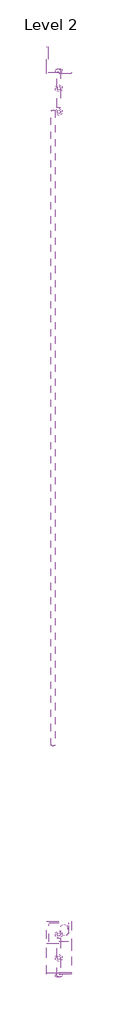
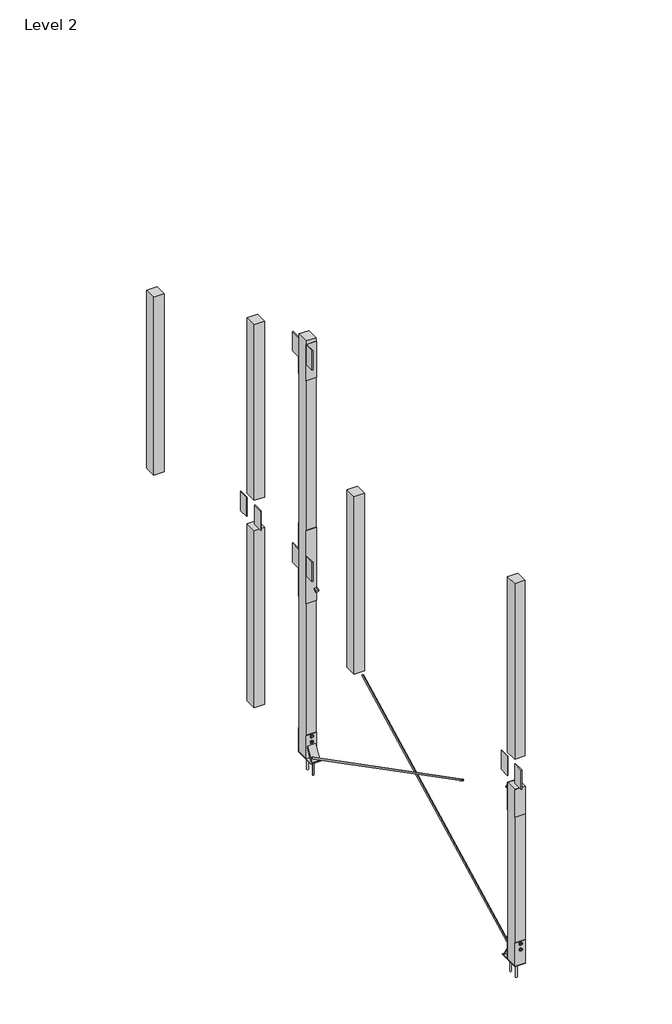
# One storey: 22 proxies, 1 column.
"""IFC4 building model written with IfcOpenShell, lengths in millimetres."""

import ifcopenshell
import ifcopenshell.guid

model = None  # the IFC model being written
_history = None  # IfcOwnerHistory: only IFC2X3 demands one
_inside = {}  # id of a spatial element -> (the spatial element, [elements in it])
_under = {}  # id of a project, library or spatial element -> (it, [spatial elements below it])
_declared = {}  # id of a project -> (the project, [libraries it declares])
_typed = {}  # id of a type object -> (the type object, [elements of that type])
_made_of = {}  # id of a material, layer set ... -> (it, [elements and type objects made of it])


def new_model(schema):
    """Start an empty IFC model of exactly this schema.

    Asked for "IFC4X3", IfcOpenShell would pick the latest addendum, in which some entities
    have other attributes; the version numbers below select the first issue.
    IFC2X3 requires an IfcOwnerHistory on every rooted entity: one is made here for all.
    """
    global model, _history
    if schema == "IFC4X3":
        model = ifcopenshell.file(schema_version=(4, 3, 0, 0))
    else:
        model = ifcopenshell.file(schema=schema)
    _inside.clear()
    _under.clear()
    _declared.clear()
    _typed.clear()
    _made_of.clear()
    _history = None
    if model.schema == "IFC2X3":
        org = make("IfcOrganization", Name="unknown")
        user = make(
            "IfcPersonAndOrganization",
            ThePerson=make("IfcPerson", FamilyName="unknown"),
            TheOrganization=org,
        )
        app = make(
            "IfcApplication",
            ApplicationDeveloper=org,
            Version="unknown",
            ApplicationFullName="unknown",
            ApplicationIdentifier="unknown",
        )
        _history = make(
            "IfcOwnerHistory",
            OwningUser=user,
            OwningApplication=app,
            ChangeAction="ADDED",
            CreationDate=0,
        )
    return model


def make(cls, **values):
    """One entity of the class cls with the attributes given. An attribute that is None is left unset."""
    return model.create_entity(
        cls, **{name: value for name, value in values.items() if value is not None}
    )


def rooted(cls, **values):
    """An entity with a GlobalId (a new one), such as an element, a storey or a relation."""
    return make(cls, GlobalId=ifcopenshell.guid.new(), OwnerHistory=_history, **values)


def si_unit(unit_type, name, prefix=None):
    """IfcSIUnit, for example si_unit("LENGTHUNIT", "METRE", prefix="MILLI")."""
    return make("IfcSIUnit", UnitType=unit_type, Prefix=prefix, Name=name)


def assignment(units):
    """IfcUnitAssignment: the units of a project."""
    return None if units is None else make("IfcUnitAssignment", Units=units)


def point(xyz):
    """IfcCartesianPoint."""
    return None if xyz is None else make("IfcCartesianPoint", Coordinates=xyz)


def direction(xyz):
    """IfcDirection."""
    return None if xyz is None else make("IfcDirection", DirectionRatios=xyz)


def frame(location, z_axis=None, x_axis=None):
    """IfcAxis2Placement3D, a coordinate frame: its origin and axes. An axis left out is left unset."""
    return make(
        "IfcAxis2Placement3D",
        Location=point(location),
        Axis=direction(z_axis),
        RefDirection=direction(x_axis),
    )


def frame_2d(location, x_axis=None):
    """IfcAxis2Placement2D, a coordinate frame in the plane: its origin and x axis."""
    return make(
        "IfcAxis2Placement2D", Location=point(location), RefDirection=direction(x_axis)
    )


def origin():
    """The frame at (0, 0, 0) with its axes left unset."""
    return frame((0.0, 0.0, 0.0))


def place(relative_to, where):
    """IfcLocalPlacement: puts the frame where relative to a parent placement (None: the world)."""
    return make(
        "IfcLocalPlacement", PlacementRelTo=relative_to, RelativePlacement=where
    )


def context(
    kind, dimensions, precision=None, world=None, true_north=None, identifier=None
):
    """IfcGeometricRepresentationContext, for example the 3D "Model" context."""
    return make(
        "IfcGeometricRepresentationContext",
        ContextIdentifier=identifier,
        ContextType=kind,
        CoordinateSpaceDimension=dimensions,
        Precision=precision,
        WorldCoordinateSystem=world,
        TrueNorth=true_north,
    )


def project(units=None, contexts=None):
    """IfcProject with its units and contexts."""
    return rooted(
        "IfcProject",
        Name="project",
        RepresentationContexts=contexts,
        UnitsInContext=assignment(units),
    )


def spatial(cls, under=None, at=None, **own):
    """A site, building, storey or space (cls), placed at a placement, below another one or the project."""
    s = rooted(cls, ObjectPlacement=at, **own)
    if under is not None:
        _under.setdefault(under.id(), (under, []))[1].append(s)
    return s


def polyline(points):
    """IfcPolyline through the points."""
    return make("IfcPolyline", Points=[point(p) for p in points])


def circle_curve(where, radius):
    """IfcCircle in the frame where."""
    return make("IfcCircle", Position=where, Radius=radius)


def trimmed(basis, trim1, trim2, sense, master):
    """IfcTrimmedCurve: the piece of a basis curve between two trims."""
    return make(
        "IfcTrimmedCurve",
        BasisCurve=basis,
        Trim1=trim1,
        Trim2=trim2,
        SenseAgreement=sense,
        MasterRepresentation=master,
    )


def segment(curve, same_sense, transition):
    """IfcCompositeCurveSegment."""
    return make(
        "IfcCompositeCurveSegment",
        Transition=transition,
        SameSense=same_sense,
        ParentCurve=curve,
    )


def composite_curve(segments, self_intersect=None):
    """IfcCompositeCurve: segments joined end to end."""
    return make("IfcCompositeCurve", Segments=segments, SelfIntersect=self_intersect)


def outline(outer, holes=None, kind="AREA"):
    """IfcArbitraryClosedProfileDef: a profile drawn as a closed curve; with holes, ...WithVoids."""
    if holes is None:
        return make("IfcArbitraryClosedProfileDef", ProfileType=kind, OuterCurve=outer)
    return make(
        "IfcArbitraryProfileDefWithVoids",
        ProfileType=kind,
        OuterCurve=outer,
        InnerCurves=holes,
    )


def extrude(swept, where, along, depth):
    """IfcExtrudedAreaSolid: the profile swept, set in the frame where, extruded along a direction by depth."""
    return make(
        "IfcExtrudedAreaSolid",
        SweptArea=swept,
        Position=where,
        ExtrudedDirection=direction(along),
        Depth=depth,
    )


def faces_of(points, faces, orient=None, outer=None):
    """IfcFace entities. A face is a list of loops; a loop is a list of indices into points, from 0.

    orient and outer hold one flag for each loop. By default every Orientation is true, the
    first loop of a face is its IfcFaceOuterBound and the others are IfcFaceBound.
    """
    made = []
    for i, loops in enumerate(faces):
        bounds = []
        for j, loop in enumerate(loops):
            is_outer = j == 0 if outer is None else outer[i][j]
            bounds.append(
                make(
                    "IfcFaceOuterBound" if is_outer else "IfcFaceBound",
                    Bound=make("IfcPolyLoop", Polygon=[points[k] for k in loop]),
                    Orientation=True if orient is None else orient[i][j],
                )
            )
        made.append(make("IfcFace", Bounds=bounds))
    return made


def faceted_brep(points, faces, orient=None, outer=None, voids=None):
    """IfcFacetedBrep: a solid bounded by flat faces; with voids (closed shells), ...WithVoids."""
    shared = [point(p) for p in points]
    hull = make("IfcClosedShell", CfsFaces=faces_of(shared, faces, orient, outer))
    if voids is None:
        return make("IfcFacetedBrep", Outer=hull)
    return make(
        "IfcFacetedBrepWithVoids",
        Outer=hull,
        Voids=[
            make(cls, CfsFaces=faces_of(shared, fs, o, b)) for cls, fs, o, b in voids
        ],
    )


def shape(context_of_items, identifier, shape_type, items):
    """IfcShapeRepresentation: the items that make up one representation, for example the "Body"."""
    return make(
        "IfcShapeRepresentation",
        ContextOfItems=context_of_items,
        RepresentationIdentifier=identifier,
        RepresentationType=shape_type,
        Items=items,
    )


def source(mapping_origin, context_of_items, identifier, shape_type, items):
    """IfcRepresentationMap: a shape defined once, which mapped items show again and again."""
    return make(
        "IfcRepresentationMap",
        MappingOrigin=mapping_origin,
        MappedRepresentation=shape(context_of_items, identifier, shape_type, items),
    )


def transform(
    local_origin,
    x_axis=None,
    y_axis=None,
    z_axis=None,
    scale=None,
    scale2=None,
    scale3=None,
    uniform=True,
):
    """IfcCartesianTransformationOperator3D, or its non-uniform kind. x_axis, y_axis, z_axis: its Axis1, 2, 3."""
    if uniform:
        return make(
            "IfcCartesianTransformationOperator3D",
            Axis1=direction(x_axis),
            Axis2=direction(y_axis),
            LocalOrigin=point(local_origin),
            Scale=scale,
            Axis3=direction(z_axis),
        )
    return make(
        "IfcCartesianTransformationOperator3DnonUniform",
        Axis1=direction(x_axis),
        Axis2=direction(y_axis),
        LocalOrigin=point(local_origin),
        Scale=scale,
        Axis3=direction(z_axis),
        Scale2=scale2,
        Scale3=scale3,
    )


def mapped(mapping_source, mapping_target):
    """IfcMappedItem: shows the shape of a source again, moved by a transform."""
    return make(
        "IfcMappedItem", MappingSource=mapping_source, MappingTarget=mapping_target
    )


def made_of(thing, what):
    """Note that an element or type object is made of a material, layer set ...; save() writes the relation."""
    if what is not None:
        _made_of.setdefault(what.id(), (what, []))[1].append(thing)
    return thing


def element(
    cls,
    number,
    at=None,
    inside=None,
    cuts=None,
    type_object=None,
    material=None,
    context=None,
    identifier="Body",
    shape_type=None,
    held_by="IfcProductDefinitionShape",
    body=None,
    shapes=None,
    **own,
):
    """One element of the class cls, such as IfcWall. Its Tag is "e" and its number.

    at: its placement. inside: the storey or other place that contains it. cuts: it is an
    opening in that element (IfcRelVoidsElement). A single representation is given by context,
    identifier, shape_type and body (its items); several are given by shapes. held_by: the class
    of the entity that holds the representations. save() writes the other relations.
    """
    e = rooted(cls, Tag="e%d" % number, ObjectPlacement=at, **own)
    if body is not None:
        shapes = [shape(context, identifier, shape_type, body)]
    if shapes is not None:
        e.Representation = make(held_by, Representations=shapes)
    if inside is not None:
        _inside.setdefault(inside.id(), (inside, []))[1].append(e)
    if cuts is not None:
        rooted(
            "IfcRelVoidsElement", RelatingBuildingElement=cuts, RelatedOpeningElement=e
        )
    if type_object is not None:
        _typed.setdefault(type_object.id(), (type_object, []))[1].append(e)
    return made_of(e, material)


def aggregate(whole, parts):
    """IfcRelAggregates: a whole, such as a stair, and the parts it consists of."""
    return rooted("IfcRelAggregates", RelatingObject=whole, RelatedObjects=parts)


def save(model, path):
    """Write the relations noted so far, then the file.

    IfcRelAggregates (storeys below a building ...), IfcRelContainedInSpatialStructure (elements
    in a storey), IfcRelDefinesByType, IfcRelAssociatesMaterial and IfcRelDeclares: one each for
    every whole, place, type object, material and project.
    """
    for whole, parts in _under.values():
        aggregate(whole, parts)
    for where, things in _inside.values():
        rooted(
            "IfcRelContainedInSpatialStructure",
            RelatedElements=things,
            RelatingStructure=where,
        )
    for kind, things in _typed.values():
        rooted("IfcRelDefinesByType", RelatedObjects=things, RelatingType=kind)
    for what, things in _made_of.values():
        rooted("IfcRelAssociatesMaterial", RelatedObjects=things, RelatingMaterial=what)
    for by, libraries in _declared.values():
        rooted("IfcRelDeclares", RelatingContext=by, RelatedDefinitions=libraries)
    model.write(path)


def plane_surface(at):
    """IfcPlane: the flat surface through the origin of the frame at, square to its z axis."""
    return make("IfcPlane", Position=at)


def extruded_surface(curve, direction_of_extrusion, depth):
    """IfcSurfaceOfLinearExtrusion: the curve pushed along a direction by depth."""
    return make(
        "IfcSurfaceOfLinearExtrusion",
        SweptCurve=make("IfcArbitraryOpenProfileDef", ProfileType="CURVE", Curve=curve),
        ExtrudedDirection=direction(direction_of_extrusion),
        Depth=depth,
    )


def advanced_brep(points, edges, surfaces, faces):
    """IfcAdvancedBrep: a solid bounded by faces that lie on surfaces and meet in shared edges.

    An edge is (start, end): straight between two places in points (the first is 0);
    or (start, end, curve); or (start, end, curve, False) where it runs against its curve.
    A face is (place in surfaces, loops), or (place, loops, False) where it looks against
    its surface's normal. A loop lists edges by number (the first is 1), with a minus sign
    where the edge is run from its end to its start. The first loop is the outer one.
    """
    corners = [point(p) for p in points]
    vertices = [make("IfcVertexPoint", VertexGeometry=c) for c in corners]
    made = []
    for start, end, *more in edges:
        made.append(
            make(
                "IfcEdgeCurve",
                EdgeStart=vertices[start],
                EdgeEnd=vertices[end],
                EdgeGeometry=more[0] if more else make("IfcPolyline", Points=[corners[start], corners[end]]),
                SameSense=more[1] if len(more) > 1 else True,
            )
        )
    hull = []
    for where, loops, *sense in faces:
        bounds = []
        for j, loop in enumerate(loops):
            ring = [make("IfcOrientedEdge", EdgeElement=made[abs(k) - 1], Orientation=k > 0) for k in loop]
            bounds.append(
                make(
                    "IfcFaceOuterBound" if j == 0 else "IfcFaceBound",
                    Bound=make("IfcEdgeLoop", EdgeList=ring),
                    Orientation=True,
                )
            )
        hull.append(make("IfcAdvancedFace", Bounds=bounds, FaceSurface=surfaces[where], SameSense=sense[0] if sense else True))
    return make("IfcAdvancedBrep", Outer=make("IfcClosedShell", CfsFaces=hull))


def generic_models_100_generic_models_75_5ab5e8ab(model_context):
    return source(origin(), model_context, "Body", "SweptSolid", [
        extrude(outline(polyline([(266616.6501684, 31991.9073871), (266635.7001684, 31991.9073871), (266645.2251684, 31975.4096032), (266635.7001684, 31958.9118192), (266616.6501684, 31958.9118192), (266607.1251684, 31975.4096032), (266616.6501684, 31991.9073871)])), frame((0.0, 35373.9582942, 0.0), z_axis=(0.0, 1.0, 0.0), x_axis=(0.0, 0.0, 1.0)), (0.0, 0.0, 1.0), 13.49375),
        extrude(outline(polyline([(266616.6501684, 31991.9073871), (266635.7001684, 31991.9073871), (266645.2251684, 31975.4096032), (266635.7001684, 31958.9118192), (266616.6501684, 31958.9118192), (266607.1251684, 31975.4096032), (266616.6501684, 31991.9073871)])), frame((0.0, 35192.1895442, 0.0), z_axis=(0.0, 1.0, 0.0), x_axis=(0.0, 0.0, 1.0)), (0.0, 0.0, 1.0), 13.49375),
    ])


def generic_models_103_generic_models_73_86a274db(model_context):
    return source(origin(), model_context, "Body", "SweptSolid", [
        extrude(outline(polyline([(32040.4971032, 30858.4781612), (32040.4971032, 30850.5406612), (31910.3221032, 30850.5406612), (31910.3221032, 30858.4781612), (32040.4971032, 30858.4781612)])), frame((0.0, 0.0, 268388.9485545), z_axis=(0.0, 0.0, 1.0), x_axis=(1.0, 0.0, 0.0)), (0.0, 0.0, 1.0), 360.5139455),
        extrude(outline(polyline([(32040.4971032, 30698.1406612), (32040.4971032, 30690.2031612), (31910.3221032, 30690.2031612), (31910.3221032, 30698.1406612), (32040.4971032, 30698.1406612)])), frame((0.0, 0.0, 268388.9485545), z_axis=(0.0, 0.0, 1.0), x_axis=(1.0, 0.0, 0.0)), (0.0, 0.0, 1.0), 360.5139455),
        extrude(outline(polyline([(32040.4971032, 30858.4781612), (32040.4971032, 30850.5406612), (31910.3221032, 30850.5406612), (31910.3221032, 30858.4781612), (32040.4971032, 30858.4781612)])), frame((0.0, 0.0, 266422.1875), z_axis=(0.0, 0.0, 1.0), x_axis=(1.0, 0.0, 0.0)), (0.0, 0.0, 1.0), 304.8),
        extrude(outline(polyline([(32040.4971032, 30698.1406612), (32040.4971032, 30690.2031612), (31910.3221032, 30690.2031612), (31910.3221032, 30698.1406612), (32040.4971032, 30698.1406612)])), frame((0.0, 0.0, 266422.1875), z_axis=(0.0, 0.0, 1.0), x_axis=(1.0, 0.0, 0.0)), (0.0, 0.0, 1.0), 304.8),
    ])


def generic_models_106_generic_models_75_9af4e480(model_context):
    return source(origin(), model_context, "Body", "SweptSolid", [
        extrude(outline(polyline([(266616.6501684, 31991.9073871), (266635.7001684, 31991.9073871), (266645.2251684, 31975.4096032), (266635.7001684, 31958.9118192), (266616.6501684, 31958.9118192), (266607.1251684, 31975.4096032), (266616.6501684, 31991.9073871)])), frame((0.0, 30858.4781612, 0.0), z_axis=(0.0, 1.0, 0.0), x_axis=(0.0, 0.0, 1.0)), (0.0, 0.0, 1.0), 13.49375),
        extrude(outline(polyline([(266616.6501684, 31991.9073871), (266635.7001684, 31991.9073871), (266645.2251684, 31975.4096032), (266635.7001684, 31958.9118192), (266616.6501684, 31958.9118192), (266607.1251684, 31975.4096032), (266616.6501684, 31991.9073871)])), frame((0.0, 30676.7094112, 0.0), z_axis=(0.0, 1.0, 0.0), x_axis=(0.0, 0.0, 1.0)), (0.0, 0.0, 1.0), 13.49375),
    ])


def generic_models_107_generic_models_75_b10bc95d(model_context):
    return source(origin(), model_context, "Body", "SweptSolid", [
        extrude(outline(composite_curve([segment(trimmed(circle_curve(frame_2d((268495.4625, 31975.4096032)), 9.525), [point((268495.4625, 31965.8846032))], [point((268495.4625, 31984.9346032))], False, "CARTESIAN"), True, "CONTINUOUS"), segment(trimmed(circle_curve(frame_2d((268495.4625, 31975.4096032)), 9.525), [point((268495.4625, 31984.9346032))], [point((268495.4625, 31965.8846032))], False, "CARTESIAN"), True, "CONTINUOUS")], self_intersect=False)), frame((0.0, 30672.7406612, 0.0), z_axis=(0.0, 1.0, 0.0), x_axis=(0.0, 0.0, 1.0)), (0.0, 0.0, 1.0), 203.2),
    ])


def generic_models_116_generic_models_73_6fc075d3(model_context):
    return source(origin(), model_context, "Body", "SweptSolid", [
        extrude(outline(polyline([(30957.3619232, 266422.1875), (30940.0029838, 266422.1875), (30858.4781612, 266552.9810297), (30858.4781612, 266583.1406619), (30957.3619232, 266422.1875)])), frame((31924.6096032, 0.0, 0.0), z_axis=(1.0, 0.0, 0.0), x_axis=(0.0, 1.0, 0.0)), (0.0, 0.0, 1.0), 101.6),
        extrude(outline(polyline([(35106.7995322, 266422.1875), (35205.6832942, 266583.1406619), (35205.6832942, 266552.9810297), (35124.1584716, 266422.1875), (35106.7995322, 266422.1875)])), frame((31924.6096032, 0.0, 0.0), z_axis=(1.0, 0.0, 0.0), x_axis=(0.0, 1.0, 0.0)), (0.0, 0.0, 1.0), 101.6),
    ])


def generic_models_120_generic_models_73_a88c3939(model_context):
    return source(origin(), model_context, "Body", "SweptSolid", [
        extrude(outline(polyline([(32040.4971032, 30964.2606313), (32040.4971032, 30690.2031612), (31910.3221032, 30690.2031612), (31910.3221032, 30964.2606313), (32040.4971032, 30964.2606313)])), frame((0.0, 0.0, 266414.25), z_axis=(0.0, 0.0, 1.0), x_axis=(1.0, 0.0, 0.0)), (0.0, 0.0, 1.0), 7.9375),
        extrude(outline(polyline([(32040.4971032, 35373.9582942), (32040.4971032, 35100.8368035), (31910.3221032, 35100.8368035), (31910.3221032, 35373.9582942), (32040.4971032, 35373.9582942)])), frame((0.0, 0.0, 266414.25), z_axis=(0.0, 0.0, 1.0), x_axis=(1.0, 0.0, 0.0)), (0.0, 0.0, 1.0), 7.9375),
    ])


def generic_models_139_generic_models_119_bb35afc2(model_context):
    return source(origin(), model_context, "Body", "AdvancedBrep", [
        advanced_brep(
        [(32003.9965778, 30877.5659964, 266463.8403309), (32003.9965778, 30886.2933954, 266446.9070794), (32002.4450787, 34140.039121, 268145.3192042), (32002.4450787, 34148.76652, 268128.3859527)],
        [
            (0, 1, circle_curve(frame((32003.9965778, 30881.9296959, 266455.3737052), z_axis=(0.0, -0.8888845937971532, -0.4581311808969894), x_axis=(0.0, 0.4581311808969894, -0.8888845937971532)), 9.525)),
            (1, 0, circle_curve(frame((32003.9965778, 30881.9296959, 266455.3737052), z_axis=(0.0, -0.8888845937971532, -0.4581311808969894), x_axis=(0.0, 0.4581311808969894, -0.8888845937971532)), 9.525)),
            (2, 3, circle_curve(frame((32002.4450787, 34144.4028205, 268136.8525784), z_axis=(0.0, 0.8888845937971532, 0.4581311808969894), x_axis=(0.0, 0.4581311808969894, -0.8888845937971532)), 9.525)),
            (3, 2, circle_curve(frame((32002.4450787, 34144.4028205, 268136.8525784), z_axis=(0.0, 0.8888845937971532, 0.4581311808969894), x_axis=(0.0, 0.4581311808969894, -0.8888845937971532)), 9.525)),
            (3, 1),
            (0, 2),
        ],
        [
            plane_surface(frame((32003.9965778, 30881.9296959, 266455.3737052), z_axis=(0.0, -0.8888845937971532, -0.4581311808969894), x_axis=(-1.0, 0.0, 0.0))),
            plane_surface(frame((32002.4450787, 34144.4028205, 268136.8525784), z_axis=(0.0, 0.8888845937971532, 0.4581311808969894), x_axis=(-1.0, 0.0, 0.0))),
            extruded_surface(trimmed(circle_curve(frame((32002.4450787, 34144.4028205, 268136.8525784), z_axis=(0.0, -0.8888845937971532, -0.4581311808969894), x_axis=(0.0, 0.4581311808969894, -0.8888845937971532)), 9.525), [point((32002.4450787, 34140.039121, 268145.3192042))], [point((32002.4450787, 34148.76652, 268128.3859527))], True, "CARTESIAN"), (1.55149910000182, -3262.473124600001, -1681.478873200016), 3670.3003278893602),
            extruded_surface(trimmed(circle_curve(frame((32002.4450787, 34144.4028205, 268136.8525784), z_axis=(0.0, -0.8888845937971532, -0.4581311808969894), x_axis=(0.0, 0.4581311808969894, -0.8888845937971532)), 9.525), [point((32002.4450787, 34148.76652, 268128.3859527))], [point((32002.4450787, 34140.039121, 268145.3192042))], True, "CARTESIAN"), (1.55149910000182, -3262.473124600001, -1681.478873200016), 3670.3003278893602),
        ],
        [
            (0, [[1, 2]]),
            (1, [[3, 4]]),
            (2, [[-4, 5, -1, 6]]),
            (3, [[-3, -6, -2, -5]]),
        ],
    ),
        advanced_brep(
        [(31945.3483901, 35168.4634288, 266435.1980333), (31945.3483901, 35177.2143812, 266452.1191247), (31945.2937775, 31874.4909796, 268138.7167634), (31945.2937775, 31883.241932, 268155.6378548)],
        [
            (0, 1, circle_curve(frame((31945.3483901, 35172.838905, 266443.658579), z_axis=(0.0, 0.8882462650221944, -0.459367579041144), x_axis=(0.0, 0.459367579041144, 0.8882462650221944)), 9.525)),
            (1, 0, circle_curve(frame((31945.3483901, 35172.838905, 266443.658579), z_axis=(0.0, 0.8882462650221944, -0.459367579041144), x_axis=(0.0, 0.459367579041144, 0.8882462650221944)), 9.525)),
            (2, 3, circle_curve(frame((31945.2937775, 31878.8664558, 268147.1773091), z_axis=(0.0, -0.8882462650221944, 0.459367579041144), x_axis=(0.0, 0.459367579041144, 0.8882462650221944)), 9.525)),
            (3, 2, circle_curve(frame((31945.2937775, 31878.8664558, 268147.1773091), z_axis=(0.0, -0.8882462650221944, 0.459367579041144), x_axis=(0.0, 0.459367579041144, 0.8882462650221944)), 9.525)),
            (3, 1),
            (0, 2),
        ],
        [
            plane_surface(frame((31945.3483901, 35172.838905, 266443.658579), z_axis=(0.0, 0.8882462650221944, -0.459367579041144), x_axis=(-1.0, 0.0, 0.0))),
            plane_surface(frame((31945.2937775, 31878.8664558, 268147.1773091), z_axis=(0.0, -0.8882462650221944, 0.459367579041144), x_axis=(-1.0, 0.0, 0.0))),
            extruded_surface(trimmed(circle_curve(frame((31945.2937775, 31878.8664558, 268147.1773091), z_axis=(0.0, 0.8882462650221944, -0.459367579041144), x_axis=(0.0, 0.459367579041144, 0.8882462650221944)), 9.525), [point((31945.2937775, 31874.4909796, 268138.7167634))], [point((31945.2937775, 31883.241932, 268155.6378548))], True, "CARTESIAN"), (0.05461260000083712, 3293.9724491999987, -1703.5187301000115), 3708.400000387327),
            extruded_surface(trimmed(circle_curve(frame((31945.2937775, 31878.8664558, 268147.1773091), z_axis=(0.0, 0.8882462650221944, -0.459367579041144), x_axis=(0.0, 0.459367579041144, 0.8882462650221944)), 9.525), [point((31945.2937775, 31883.241932, 268155.6378548))], [point((31945.2937775, 31874.4909796, 268138.7167634))], True, "CARTESIAN"), (0.05461260000083712, 3293.9724491999987, -1703.5187301000115), 3708.400000387327),
        ],
        [
            (0, [[1, 2]]),
            (1, [[3, 4]]),
            (2, [[-4, 5, -1, 6]]),
            (3, [[-3, -6, -2, -5]]),
        ],
    ),
    ])


def generic_models_222_generic_models_75_2b5840a4(model_context):
    return source(origin(), model_context, "Body", "SweptSolid", [
        extrude(outline(composite_curve([segment(trimmed(circle_curve(frame_2d((31975.4096032, 30896.6257369)), 9.525), [point((31965.8846032, 30896.6257369))], [point((31984.9346032, 30896.6257369))], False, "CARTESIAN"), True, "CONTINUOUS"), segment(trimmed(circle_curve(frame_2d((31975.4096032, 30896.6257369)), 9.525), [point((31984.9346032, 30896.6257369))], [point((31965.8846032, 30896.6257369))], False, "CARTESIAN"), True, "CONTINUOUS")], self_intersect=False)), frame((0.0, 0.0, 266211.05), z_axis=(0.0, 0.0, 1.0), x_axis=(1.0, 0.0, 0.0)), (0.0, 0.0, 1.0), 228.6),
    ])


def generic_models_223_generic_models_75_c2a9037b(model_context):
    return source(origin(), model_context, "Body", "SweptSolid", [
        extrude(outline(polyline([(31991.9073871, 30887.1007369), (31975.4096032, 30877.5757369), (31958.9118192, 30887.1007369), (31958.9118192, 30906.1507369), (31975.4096032, 30915.6757369), (31991.9073871, 30906.1507369), (31991.9073871, 30887.1007369)])), frame((0.0, 0.0, 266422.1875), z_axis=(0.0, 0.0, 1.0), x_axis=(1.0, 0.0, 0.0)), (0.0, 0.0, 1.0), 13.49375),
    ])


def generic_models_93_generic_models_73_0b4a4ac0(model_context):
    return source(origin(), model_context, "Body", "SweptSolid", [
        extrude(outline(polyline([(31910.3221032, 30691.7906612), (31918.2596032, 30691.7906612), (31918.2596032, 30560.0281612), (31910.3221032, 30560.0281612), (31910.3221032, 30691.7906612)])), frame((0.0, 0.0, 268836.775), z_axis=(0.0, 0.0, 1.0), x_axis=(1.0, 0.0, 0.0)), (0.0, 0.0, 1.0), 254.0),
        extrude(outline(polyline([(31910.3221032, 30990.2406612), (31918.2596032, 30990.2406612), (31918.2596032, 30858.4781612), (31910.3221032, 30858.4781612), (31910.3221032, 30990.2406612)])), frame((0.0, 0.0, 268836.775), z_axis=(0.0, 0.0, 1.0), x_axis=(1.0, 0.0, 0.0)), (0.0, 0.0, 1.0), 254.0),
        extrude(outline(polyline([(31910.3221032, 36321.6957942), (31918.2596032, 36321.6957942), (31918.2596032, 36193.1082942), (31910.3221032, 36193.1082942), (31910.3221032, 36321.6957942)])), frame((0.0, 0.0, 268836.775), z_axis=(0.0, 0.0, 1.0), x_axis=(1.0, 0.0, 0.0)), (0.0, 0.0, 1.0), 254.0),
        extrude(outline(polyline([(31910.3221032, 36623.3207942), (31918.2596032, 36623.3207942), (31918.2596032, 36493.1457942), (31910.3221032, 36493.1457942), (31910.3221032, 36623.3207942)])), frame((0.0, 0.0, 268836.775), z_axis=(0.0, 0.0, 1.0), x_axis=(1.0, 0.0, 0.0)), (0.0, 0.0, 1.0), 254.0),
        extrude(outline(polyline([(31910.3221032, 35207.2707942), (31918.2596032, 35207.2707942), (31918.2596032, 35075.5082942), (31910.3221032, 35075.5082942), (31910.3221032, 35207.2707942)])), frame((0.0, 0.0, 271626.0125), z_axis=(0.0, 0.0, 1.0), x_axis=(1.0, 0.0, 0.0)), (0.0, 0.0, 1.0), 254.0),
        extrude(outline(polyline([(31910.3221032, 35505.7207942), (31918.2596032, 35505.7207942), (31918.2596032, 35373.9582942), (31910.3221032, 35373.9582942), (31910.3221032, 35505.7207942)])), frame((0.0, 0.0, 271621.25), z_axis=(0.0, 0.0, 1.0), x_axis=(1.0, 0.0, 0.0)), (0.0, 0.0, 1.0), 254.0),
        extrude(outline(polyline([(31910.3221032, 35207.2707942), (31918.2596032, 35207.2707942), (31918.2596032, 35075.5082942), (31910.3221032, 35075.5082942), (31910.3221032, 35207.2707942)])), frame((0.0, 0.0, 268836.775), z_axis=(0.0, 0.0, 1.0), x_axis=(1.0, 0.0, 0.0)), (0.0, 0.0, 1.0), 254.0),
        extrude(outline(polyline([(31910.3221032, 35505.7207942), (31918.2596032, 35505.7207942), (31918.2596032, 35373.9582942), (31910.3221032, 35373.9582942), (31910.3221032, 35505.7207942)])), frame((0.0, 0.0, 268832.0125), z_axis=(0.0, 0.0, 1.0), x_axis=(1.0, 0.0, 0.0)), (0.0, 0.0, 1.0), 254.0),
        extrude(outline(polyline([(32040.4971032, 35213.6207942), (32040.4971032, 35205.6832942), (31910.3221032, 35205.6832942), (31910.3221032, 35213.6207942), (32040.4971032, 35213.6207942)])), frame((0.0, 0.0, 266422.1875), z_axis=(0.0, 0.0, 1.0), x_axis=(1.0, 0.0, 0.0)), (0.0, 0.0, 1.0), 304.8),
        extrude(outline(polyline([(32040.4971032, 35373.9582942), (32040.4971032, 35366.0207942), (31910.3221032, 35366.0207942), (31910.3221032, 35373.9582942), (32040.4971032, 35373.9582942)])), frame((0.0, 0.0, 266422.1875), z_axis=(0.0, 0.0, 1.0), x_axis=(1.0, 0.0, 0.0)), (0.0, 0.0, 1.0), 304.8),
        extrude(outline(polyline([(32040.4971032, 35213.6207942), (32040.4971032, 35205.6832942), (31910.3221032, 35205.6832942), (31910.3221032, 35213.6207942), (32040.4971032, 35213.6207942)])), frame((0.0, 0.0, 271406.9375), z_axis=(0.0, 0.0, 1.0), x_axis=(1.0, 0.0, 0.0)), (0.0, 0.0, 1.0), 473.075),
        extrude(outline(polyline([(32040.4971032, 35373.9582942), (32040.4971032, 35366.0207942), (31910.3221032, 35366.0207942), (31910.3221032, 35373.9582942), (32040.4971032, 35373.9582942)])), frame((0.0, 0.0, 271406.9375), z_axis=(0.0, 0.0, 1.0), x_axis=(1.0, 0.0, 0.0)), (0.0, 0.0, 1.0), 473.075),
        extrude(outline(polyline([(32040.4971032, 35373.9582942), (32040.4971032, 35366.0207942), (31910.3221032, 35366.0207942), (31910.3221032, 35373.9582942), (32040.4971032, 35373.9582942)])), frame((0.0, 0.0, 268465.3), z_axis=(0.0, 0.0, 1.0), x_axis=(1.0, 0.0, 0.0)), (0.0, 0.0, 1.0), 965.2),
        extrude(outline(polyline([(32040.4971032, 35213.6207942), (32040.4971032, 35205.6832942), (31910.3221032, 35205.6832942), (31910.3221032, 35213.6207942), (32040.4971032, 35213.6207942)])), frame((0.0, 0.0, 268465.3), z_axis=(0.0, 0.0, 1.0), x_axis=(1.0, 0.0, 0.0)), (0.0, 0.0, 1.0), 965.2),
    ])


def generic_models_96_generic_models_119_cda3f510(model_context):
    return source(origin(), model_context, "Body", "SolidModel", [
        faceted_brep([(31987.4987939, 30893.1483324, 266471.7687657), (31987.4987939, 30901.8757314, 266454.8355142), (32003.9965778, 30906.2394309, 266446.3688884), (32020.4943618, 30901.8757314, 266454.8355142), (32020.4943618, 30893.1483324, 266471.7687657), (32003.9965778, 30888.7846329, 266480.2353914), (31985.9472947, 30934.9577151, 266493.3173244), (32002.4450787, 30930.5940156, 266501.7839502), (32018.9428626, 30934.9577151, 266493.3173244), (32018.9428626, 30943.6851141, 266476.3840729), (32002.4450787, 30948.0488136, 266467.9174471), (31985.9472947, 30943.6851141, 266476.3840729)], [[[0, 1, 2, 3, 4, 5]], [[6, 7, 8, 9, 10, 11]], [[6, 11, 1, 0]], [[11, 10, 2, 1]], [[10, 9, 3, 2]], [[9, 8, 4, 3]], [[8, 7, 5, 4]], [[7, 6, 0, 5]]]),
        faceted_brep([(31956.3469127, 30934.4369056, 268642.8051671), (31956.3469127, 30928.6029373, 268631.5244396), (31945.3483901, 30925.6859532, 268625.8840758), (31934.3498675, 30928.6029373, 268631.5244396), (31934.3498675, 30934.4369056, 268642.8051671), (31945.3483901, 30937.3538897, 268648.4455309), (31956.2923001, 30892.5813314, 268664.4512968), (31945.2937775, 30895.4983155, 268670.0916606), (31934.2952549, 30892.5813314, 268664.4512968), (31934.2952549, 30886.7473631, 268653.1705692), (31945.2937775, 30883.830379, 268647.5302054), (31956.2923001, 30886.7473631, 268653.1705692)], [[[0, 1, 2, 3, 4, 5]], [[6, 7, 8, 9, 10, 11]], [[6, 11, 1, 0]], [[11, 10, 2, 1]], [[10, 9, 3, 2]], [[9, 8, 4, 3]], [[8, 7, 5, 4]], [[7, 6, 0, 5]]]),
        extrude(outline(polyline([(-9.525, 16.4977839), (9.5249999, 16.4977839), (19.0499999, 0.0), (9.5249999, -16.497784), (-9.525, -16.497784), (-19.0500001, 0.0), (-9.525, 16.4977839)])), frame((32003.9965778, 35128.3976646, 268644.0035888), z_axis=(0.0, 0.8888845937971597, 0.45813118089697674), x_axis=(0.0, 0.45813118089697674, -0.8888845937971597)), (0.0, 0.0, 1.0), 44.45),
        faceted_brep([(31956.3469127, 35161.0252375, 266456.9170821), (31956.3469127, 35155.1912692, 266445.6363545), (31945.3483901, 35152.2742851, 266439.9959907), (31934.3498675, 35155.1912692, 266445.6363545), (31934.3498675, 35161.0252375, 266456.9170821), (31945.3483901, 35163.9422216, 266462.5574459), (31956.2923001, 35121.542691, 266477.335971), (31945.2937775, 35124.4596751, 266482.9763347), (31934.2952549, 35121.542691, 266477.335971), (31934.2952549, 35115.7087227, 266466.0552434), (31945.2937775, 35112.7917386, 266460.4148796), (31956.2923001, 35115.7087227, 266466.0552434)], [[[0, 1, 2, 3, 4, 5]], [[6, 7, 8, 9, 10, 11]], [[6, 11, 1, 0]], [[11, 10, 2, 1]], [[10, 9, 3, 2]], [[9, 8, 4, 3]], [[8, 7, 5, 4]], [[7, 6, 0, 5]]]),
    ])


def columns_2_columns_2_bbcb63ce(model_context):
    return source(origin(), model_context, "Body", "SweptSolid", [
        extrude(outline(polyline([(31910.3221032, 36331.2207942), (31910.3221032, 36483.6207942), (32040.4971032, 36483.6207942), (32040.4971032, 36331.2207942), (31910.3221032, 36331.2207942)])), frame((0.0, 0.0, 269146.3375), z_axis=(0.0, 0.0, 1.0), x_axis=(1.0, 0.0, 0.0)), (0.0, 0.0, 1.0), 2316.1625),
        extrude(outline(polyline([(31910.3221032, 35213.6207942), (31910.3221032, 35366.0207942), (32040.4971032, 35366.0207942), (32040.4971032, 35213.6207942), (31910.3221032, 35213.6207942)])), frame((0.0, 0.0, 266422.1875), z_axis=(0.0, 0.0, 1.0), x_axis=(1.0, 0.0, 0.0)), (0.0, 0.0, 1.0), 5505.45),
        extrude(outline(polyline([(33159.6965778, 40668.9106612), (33159.6965778, 40821.3106612), (33289.8715778, 40821.3106612), (33289.8715778, 40668.9106612), (33159.6965778, 40668.9106612)])), frame((0.0, 0.0, 266414.25), z_axis=(0.0, 0.0, 1.0), x_axis=(1.0, 0.0, 0.0)), (0.0, 0.0, 1.0), 2343.15),
        extrude(outline(polyline([(33159.6965778, 36331.2207942), (33159.6965778, 36483.6207942), (33289.8715778, 36483.6207942), (33289.8715778, 36331.2207942), (33159.6965778, 36331.2207942)])), frame((0.0, 0.0, 266414.25), z_axis=(0.0, 0.0, 1.0), x_axis=(1.0, 0.0, 0.0)), (0.0, 0.0, 1.0), 2343.15),
        extrude(outline(polyline([(31911.9215778, 36331.2207942), (31911.9215778, 36483.6207942), (32042.0965778, 36483.6207942), (32042.0965778, 36331.2207942), (31911.9215778, 36331.2207942)])), frame((0.0, 0.0, 266414.25), z_axis=(0.0, 0.0, 1.0), x_axis=(1.0, 0.0, 0.0)), (0.0, 0.0, 1.0), 2335.2125),
        extrude(outline(polyline([(31910.3221032, 30698.1406612), (31910.3221032, 30850.5406612), (32040.4971032, 30850.5406612), (32040.4971032, 30698.1406612), (31910.3221032, 30698.1406612)])), frame((0.0, 0.0, 269146.3375), z_axis=(0.0, 0.0, 1.0), x_axis=(1.0, 0.0, 0.0)), (0.0, 0.0, 1.0), 2316.1625),
        extrude(outline(polyline([(31911.9215778, 30698.1406612), (31911.9215778, 30850.5406612), (32042.0965778, 30850.5406612), (32042.0965778, 30698.1406612), (31911.9215778, 30698.1406612)])), frame((0.0, 0.0, 266422.1875), z_axis=(0.0, 0.0, 1.0), x_axis=(1.0, 0.0, 0.0)), (0.0, 0.0, 1.0), 2327.275),
    ])


model = new_model("IFC4")

# Units and contexts
model_context = context("Model", 3, world=origin())
ifc_project = project(units=[si_unit("LENGTHUNIT", "METRE", prefix="MILLI")], contexts=[model_context])

# Site, building, storey
site = spatial("IfcSite", under=ifc_project)
building = spatial("IfcBuilding", under=site)
storey = spatial("IfcBuildingStorey", under=building, Name="Level 2", Elevation=3048.0)

# Proxies
placement = place(None, origin())
generic_models_100_generic_models_75_shape = generic_models_100_generic_models_75_5ab5e8ab(model_context)
element("IfcBuildingElementProxy", 1, Name="Generic Models 100 : Generic Models 75", ObjectType="Generic Models 100 : Generic Models 75", at=placement, inside=storey, context=model_context, shape_type="MappedRepresentation", body=[
    mapped(generic_models_100_generic_models_75_shape, transform((0.0, 0.0, 76.2), x_axis=(1.0, 0.0, 0.0), y_axis=(0.0, 1.0, 0.0), z_axis=(0.0, 0.0, 1.0))),
])
generic_models_103_generic_models_73_shape = generic_models_103_generic_models_73_86a274db(model_context)
element("IfcBuildingElementProxy", 2, Name="Generic Models 103 : Generic Models 73", ObjectType="Generic Models 103 : Generic Models 73", at=placement, inside=storey, context=model_context, shape_type="MappedRepresentation", body=[
    mapped(generic_models_103_generic_models_73_shape, transform((0.0, 0.0, 0.0), x_axis=(1.0, 0.0, 0.0), y_axis=(0.0, 1.0, 0.0), z_axis=(0.0, 0.0, 1.0))),
])
generic_models_106_generic_models_75_shape = generic_models_106_generic_models_75_9af4e480(model_context)
element("IfcBuildingElementProxy", 3, Name="Generic Models 106 : Generic Models 75", ObjectType="Generic Models 106 : Generic Models 75", at=placement, inside=storey, context=model_context, shape_type="MappedRepresentation", body=[
    mapped(generic_models_106_generic_models_75_shape, transform((0.0, 0.0, 0.0), x_axis=(1.0, 0.0, 0.0), y_axis=(0.0, 1.0, 0.0), z_axis=(0.0, 0.0, 1.0))),
])
generic_models_107_generic_models_75_shape = generic_models_107_generic_models_75_b10bc95d(model_context)
element("IfcBuildingElementProxy", 4, Name="Generic Models 113 : Generic Models 75", ObjectType="Generic Models 113 : Generic Models 75", at=placement, inside=storey, context=model_context, shape_type="MappedRepresentation", body=[
    mapped(generic_models_107_generic_models_75_shape, transform((0.0, 0.0, -1869.2873316), x_axis=(1.0, 0.0, 0.0), y_axis=(0.0, 1.0, 0.0), z_axis=(0.0, 0.0, 1.0))),
])
generic_models_116_generic_models_73_shape = generic_models_116_generic_models_73_6fc075d3(model_context)
element("IfcBuildingElementProxy", 5, Name="Generic Models 116 : Generic Models 73", ObjectType="Generic Models 116 : Generic Models 73", at=placement, inside=storey, context=model_context, shape_type="MappedRepresentation", body=[
    mapped(generic_models_116_generic_models_73_shape, transform((0.0, 0.0, 0.0), x_axis=(1.0, 0.0, 0.0), y_axis=(0.0, 1.0, 0.0), z_axis=(0.0, 0.0, 1.0))),
])
generic_models_120_generic_models_73_shape = generic_models_120_generic_models_73_a88c3939(model_context)
element("IfcBuildingElementProxy", 6, Name="Generic Models 120 : Generic Models 73", ObjectType="Generic Models 120 : Generic Models 73", at=placement, inside=storey, context=model_context, shape_type="MappedRepresentation", body=[
    mapped(generic_models_120_generic_models_73_shape, transform((0.0, 0.0, 0.0), x_axis=(1.0, 0.0, 0.0), y_axis=(0.0, 1.0, 0.0), z_axis=(0.0, 0.0, 1.0))),
])
element("IfcBuildingElementProxy", 7, Name="Generic Models 121 : Generic Models 75", ObjectType="Generic Models 121 : Generic Models 75", at=placement, inside=storey, context=model_context, shape_type="MappedRepresentation", body=[
    mapped(generic_models_107_generic_models_75_shape, transform((0.0, 4515.480133, -1869.2873316), x_axis=(1.0, 0.0, 0.0), y_axis=(0.0, 1.0, 0.0), z_axis=(0.0, 0.0, 1.0))),
])
element("IfcBuildingElementProxy", 8, Name="Generic Models 122 : Generic Models 75", ObjectType="Generic Models 122 : Generic Models 75", at=placement, inside=storey, context=model_context, shape_type="MappedRepresentation", body=[
    mapped(generic_models_100_generic_models_75_shape, transform((0.0, 0.0, 0.0), x_axis=(1.0, 0.0, 0.0), y_axis=(0.0, 1.0, 0.0), z_axis=(0.0, 0.0, 1.0))),
])
generic_models_139_generic_models_119_shape = generic_models_139_generic_models_119_bb35afc2(model_context)
element("IfcBuildingElementProxy", 9, Name="Generic Models 139 : Generic Models 119", ObjectType="Generic Models 139 : Generic Models 119", at=placement, inside=storey, context=model_context, shape_type="MappedRepresentation", body=[
    mapped(generic_models_139_generic_models_119_shape, transform((0.0, 0.0, 0.0), x_axis=(1.0, 0.0, 0.0), y_axis=(0.0, 1.0, 0.0), z_axis=(0.0, 0.0, 1.0))),
])
element("IfcBuildingElementProxy", 10, Name="Generic Models 220 : Generic Models 75", ObjectType="Generic Models 220 : Generic Models 75", at=placement, inside=storey, context=model_context, shape_type="MappedRepresentation", body=[
    mapped(generic_models_107_generic_models_75_shape, transform((0.0, 0.0, -1793.0873316), x_axis=(1.0, 0.0, 0.0), y_axis=(0.0, 1.0, 0.0), z_axis=(0.0, 0.0, 1.0))),
])
element("IfcBuildingElementProxy", 11, Name="Generic Models 221 : Generic Models 75", ObjectType="Generic Models 221 : Generic Models 75", at=placement, inside=storey, context=model_context, shape_type="MappedRepresentation", body=[
    mapped(generic_models_106_generic_models_75_shape, transform((0.0, 0.0, 76.2), x_axis=(1.0, 0.0, 0.0), y_axis=(0.0, 1.0, 0.0), z_axis=(0.0, 0.0, 1.0))),
])
generic_models_222_generic_models_75_shape = generic_models_222_generic_models_75_2b5840a4(model_context)
element("IfcBuildingElementProxy", 12, Name="Generic Models 222 : Generic Models 75", ObjectType="Generic Models 222 : Generic Models 75", at=placement, inside=storey, context=model_context, shape_type="MappedRepresentation", body=[
    mapped(generic_models_222_generic_models_75_shape, transform((0.0, 0.0, 0.0), x_axis=(1.0, 0.0, 0.0), y_axis=(0.0, 1.0, 0.0), z_axis=(0.0, 0.0, 1.0))),
])
generic_models_223_generic_models_75_shape = generic_models_223_generic_models_75_c2a9037b(model_context)
element("IfcBuildingElementProxy", 13, Name="Generic Models 223 : Generic Models 75", ObjectType="Generic Models 223 : Generic Models 75", at=placement, inside=storey, context=model_context, shape_type="MappedRepresentation", body=[
    mapped(generic_models_223_generic_models_75_shape, transform((0.0, 0.0, 0.0), x_axis=(1.0, 0.0, 0.0), y_axis=(0.0, 1.0, 0.0), z_axis=(0.0, 0.0, 1.0))),
])
element("IfcBuildingElementProxy", 14, Name="Generic Models 224 : Generic Models 75", ObjectType="Generic Models 224 : Generic Models 75", at=placement, inside=storey, context=model_context, shape_type="MappedRepresentation", body=[
    mapped(generic_models_222_generic_models_75_shape, transform((0.0, -122.2850757, 0.0), x_axis=(1.0, 0.0, 0.0), y_axis=(0.0, 1.0, 0.0), z_axis=(0.0, 0.0, 1.0))),
])
element("IfcBuildingElementProxy", 15, Name="Generic Models 225 : Generic Models 75", ObjectType="Generic Models 225 : Generic Models 75", at=placement, inside=storey, context=model_context, shape_type="MappedRepresentation", body=[
    mapped(generic_models_223_generic_models_75_shape, transform((0.0, -122.2850757, 0.0), x_axis=(1.0, 0.0, 0.0), y_axis=(0.0, 1.0, 0.0), z_axis=(0.0, 0.0, 1.0))),
])
element("IfcBuildingElementProxy", 16, Name="Generic Models 226 : Generic Models 75", ObjectType="Generic Models 226 : Generic Models 75", at=placement, inside=storey, context=model_context, shape_type="MappedRepresentation", body=[
    mapped(generic_models_222_generic_models_75_shape, transform((0.0, 4393.1950573, 0.0), x_axis=(1.0, 0.0, 0.0), y_axis=(0.0, 1.0, 0.0), z_axis=(0.0, 0.0, 1.0))),
])
element("IfcBuildingElementProxy", 17, Name="Generic Models 227 : Generic Models 75", ObjectType="Generic Models 227 : Generic Models 75", at=placement, inside=storey, context=model_context, shape_type="MappedRepresentation", body=[
    mapped(generic_models_223_generic_models_75_shape, transform((0.0, 4393.1950573, 0.0), x_axis=(1.0, 0.0, 0.0), y_axis=(0.0, 1.0, 0.0), z_axis=(0.0, 0.0, 1.0))),
])
element("IfcBuildingElementProxy", 18, Name="Generic Models 228 : Generic Models 75", ObjectType="Generic Models 228 : Generic Models 75", at=placement, inside=storey, context=model_context, shape_type="MappedRepresentation", body=[
    mapped(generic_models_222_generic_models_75_shape, transform((0.0, 4270.9099816, 0.0), x_axis=(1.0, 0.0, 0.0), y_axis=(0.0, 1.0, 0.0), z_axis=(0.0, 0.0, 1.0))),
])
element("IfcBuildingElementProxy", 19, Name="Generic Models 229 : Generic Models 75", ObjectType="Generic Models 229 : Generic Models 75", at=placement, inside=storey, context=model_context, shape_type="MappedRepresentation", body=[
    mapped(generic_models_223_generic_models_75_shape, transform((0.0, 4270.9099816, 0.0), x_axis=(1.0, 0.0, 0.0), y_axis=(0.0, 1.0, 0.0), z_axis=(0.0, 0.0, 1.0))),
])
generic_models_93_generic_models_73_shape = generic_models_93_generic_models_73_0b4a4ac0(model_context)
element("IfcBuildingElementProxy", 20, Name="Generic Models 93 : Generic Models 73", ObjectType="Generic Models 93 : Generic Models 73", at=placement, inside=storey, context=model_context, shape_type="MappedRepresentation", body=[
    mapped(generic_models_93_generic_models_73_shape, transform((0.0, 0.0, 0.0), x_axis=(1.0, 0.0, 0.0), y_axis=(0.0, 1.0, 0.0), z_axis=(0.0, 0.0, 1.0))),
])
generic_models_96_generic_models_119_shape = generic_models_96_generic_models_119_cda3f510(model_context)
element("IfcBuildingElementProxy", 21, Name="Generic Models 96 : Generic Models 119", ObjectType="Generic Models 96 : Generic Models 119", at=placement, inside=storey, context=model_context, shape_type="MappedRepresentation", body=[
    mapped(generic_models_96_generic_models_119_shape, transform((0.0, 0.0, 0.0), x_axis=(1.0, 0.0, 0.0), y_axis=(0.0, 1.0, 0.0), z_axis=(0.0, 0.0, 1.0))),
])
element("IfcBuildingElementProxy", 22, Name="Generic Models 99 : Generic Models 75", ObjectType="Generic Models 99 : Generic Models 75", at=placement, inside=storey, context=model_context, shape_type="MappedRepresentation", body=[
    mapped(generic_models_107_generic_models_75_shape, transform((0.0, 4515.480133, -1793.0873316), x_axis=(1.0, 0.0, 0.0), y_axis=(0.0, 1.0, 0.0), z_axis=(0.0, 0.0, 1.0))),
])

# Column
columns_2_columns_2_shape = columns_2_columns_2_bbcb63ce(model_context)
element("IfcColumn", 23, ObjectType="Columns 2 : Columns 2", at=placement, inside=storey, context=model_context, shape_type="MappedRepresentation", body=[
    mapped(columns_2_columns_2_shape, transform((0.0, 0.0, 0.0), x_axis=(1.0, 0.0, 0.0), y_axis=(0.0, 1.0, 0.0), z_axis=(0.0, 0.0, 1.0))),
])

save(model, "model.ifc")

# Revit data of these elements
# Project information
#   Project Issue Date = "Issue Date"
#   Project Status = "Project Status"
#   Client Name = "Owner"
#   Project Address = "Enter address here"
#   Project Name = "Project Name"
#   Project Number = "Project Number"
# Element 1 (IfcBuildingElementProxy, "Generic Models 100 : Generic Models 75")
#   Phase Created = New Construction
# Element 2 (IfcBuildingElementProxy, "Generic Models 103 : Generic Models 73")
#   Phase Created = New Construction
#   Materials on its faces: "5/16 x 5 1/2\" x 1'-0\" SIDE PLATES  CAP\nW/ 2 3/4\"DIA. THRU BOLTS"
# Element 3 (IfcBuildingElementProxy, "Generic Models 106 : Generic Models 75")
#   Phase Created = New Construction
# Element 4 (IfcBuildingElementProxy, "Generic Models 113 : Generic Models 75")
#   Phase Created = New Construction
# Element 5 (IfcBuildingElementProxy, "Generic Models 116 : Generic Models 73")
#   Phase Created = New Construction
#   Materials on its faces: "5/8\" x 4\"PLATE"
# Element 6 (IfcBuildingElementProxy, "Generic Models 120 : Generic Models 73")
#   Phase Created = New Construction
#   Materials on its faces: "6 x 5/8\" BASE PL. W/ (2) \n5/8\" EMBEDMENT EPOXY ANCHORS"
# Element 7 (IfcBuildingElementProxy, "Generic Models 121 : Generic Models 75")
#   Phase Created = New Construction
# Element 8 (IfcBuildingElementProxy, "Generic Models 122 : Generic Models 75")
#   Phase Created = New Construction
# Element 9 (IfcBuildingElementProxy, "Generic Models 139 : Generic Models 119")
#   Phase Created = New Construction
#   Materials on its faces: "3/4\" DIA. ROD"
# Element 10 (IfcBuildingElementProxy, "Generic Models 220 : Generic Models 75")
#   Phase Created = New Construction
# Element 11 (IfcBuildingElementProxy, "Generic Models 221 : Generic Models 75")
#   Phase Created = New Construction
# Element 12 (IfcBuildingElementProxy, "Generic Models 222 : Generic Models 75")
#   Phase Created = New Construction
#   Materials on its faces: "5/8\" DIA. EPOXY ANCHOR BOLTS"
# Element 13 (IfcBuildingElementProxy, "Generic Models 223 : Generic Models 75")
#   Phase Created = New Construction
#   Materials on its faces: "5/8\" DIA. EPOXY ANCHOR BOLTS"
# Element 14 (IfcBuildingElementProxy, "Generic Models 224 : Generic Models 75")
#   Phase Created = New Construction
#   Materials on its faces: "5/8\" DIA. EPOXY ANCHOR BOLTS"
# Element 15 (IfcBuildingElementProxy, "Generic Models 225 : Generic Models 75")
#   Phase Created = New Construction
#   Materials on its faces: "5/8\" DIA. EPOXY ANCHOR BOLTS"
# Element 16 (IfcBuildingElementProxy, "Generic Models 226 : Generic Models 75")
#   Phase Created = New Construction
#   Materials on its faces: "5/8\" DIA. EPOXY ANCHOR BOLTS"
# Element 17 (IfcBuildingElementProxy, "Generic Models 227 : Generic Models 75")
#   Phase Created = New Construction
#   Materials on its faces: "5/8\" DIA. EPOXY ANCHOR BOLTS"
# Element 18 (IfcBuildingElementProxy, "Generic Models 228 : Generic Models 75")
#   Phase Created = New Construction
#   Materials on its faces: "5/8\" DIA. EPOXY ANCHOR BOLTS"
# Element 19 (IfcBuildingElementProxy, "Generic Models 229 : Generic Models 75")
#   Phase Created = New Construction
#   Materials on its faces: "5/8\" DIA. EPOXY ANCHOR BOLTS"
# Element 20 (IfcBuildingElementProxy, "Generic Models 93 : Generic Models 73")
#   Phase Created = New Construction
#   Materials on its faces: "5 1/8 x 10 x 0 5/16\" PLATE W/ 3 1\"DIA. THRU BOLTS", "5/16 x 5 1/2\" x 1'-0\" SIDE PLATES  CAP\nW/ 2 3/4\"DIA. THRU BOLTS"
# Element 21 (IfcBuildingElementProxy, "Generic Models 96 : Generic Models 119")
#   Phase Created = New Construction
# Element 22 (IfcBuildingElementProxy, "Generic Models 99 : Generic Models 75")
#   Phase Created = New Construction
# Element 23 (IfcColumn, "Columns 2 : Columns 2")
#   Phase Created = New Construction
#   Materials on its faces: "5 1/8\" x 6\" GLUELAM COLUMN"
# Materials
#   "5/16 x 5 1/2\" x 1'-0\" SIDE PLATES  CAP\nW/ 2 3/4\"DIA. THRU BOLTS": class "Metal", colour RGB 199 199 199, transparency 0, Description = "Carbon steel", Cost = 0
#   "5/8\" x 4\"PLATE": class "Metal", colour RGB 199 199 199, transparency 0, Description = "Carbon steel", Cost = 0
#   "6 x 5/8\" BASE PL. W/ (2) \n5/8\" EMBEDMENT EPOXY ANCHORS": class "Metal", colour RGB 199 199 199, transparency 0, Description = "Carbon steel", Cost = 0
#   "3/4\" DIA. ROD": class "Metal", colour RGB 199 199 199, transparency 0, Description = "Carbon steel", Cost = 0
#   "5/8\" DIA. EPOXY ANCHOR BOLTS": class "Metal", colour RGB 199 199 199, transparency 0, Description = "Carbon steel", Cost = 0
#   "5 1/8 x 10 x 0 5/16\" PLATE W/ 3 1\"DIA. THRU BOLTS": class "Metal", colour RGB 199 199 199, transparency 0, Description = "Carbon steel", Cost = 0
#   "5 1/8\" x 6\" GLUELAM COLUMN": class "Wood", colour RGB 144 113 62, transparency 0, Description = "Pinus Echinata", Cost = 0
